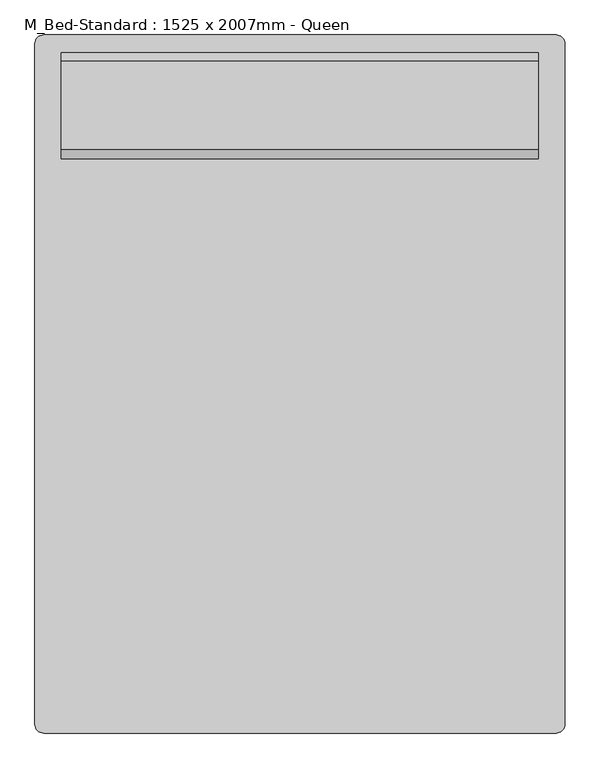
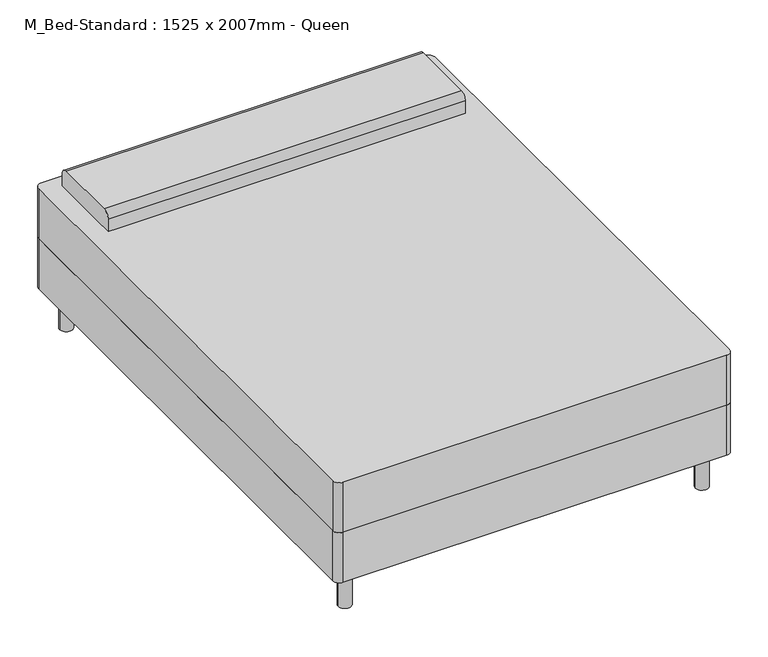
"""IFC4 building model written with IfcOpenShell, lengths in millimetres: furniture geometry, M_Bed-Standard : 1525 x 2007mm - Queen."""

import ifcopenshell
import ifcopenshell.guid

model = None  # the IFC model being written
_history = None  # IfcOwnerHistory: only IFC2X3 demands one
_inside = {}  # id of a spatial element -> (the spatial element, [elements in it])
_under = {}  # id of a project, library or spatial element -> (it, [spatial elements below it])
_declared = {}  # id of a project -> (the project, [libraries it declares])
_typed = {}  # id of a type object -> (the type object, [elements of that type])
_made_of = {}  # id of a material, layer set ... -> (it, [elements and type objects made of it])


def new_model(schema):
    """Start an empty IFC model of exactly this schema.

    Asked for "IFC4X3", IfcOpenShell would pick the latest addendum, in which some entities
    have other attributes; the version numbers below select the first issue.
    IFC2X3 requires an IfcOwnerHistory on every rooted entity: one is made here for all.
    """
    global model, _history
    if schema == "IFC4X3":
        model = ifcopenshell.file(schema_version=(4, 3, 0, 0))
    else:
        model = ifcopenshell.file(schema=schema)
    _inside.clear()
    _under.clear()
    _declared.clear()
    _typed.clear()
    _made_of.clear()
    _history = None
    if model.schema == "IFC2X3":
        org = make("IfcOrganization", Name="unknown")
        user = make(
            "IfcPersonAndOrganization",
            ThePerson=make("IfcPerson", FamilyName="unknown"),
            TheOrganization=org,
        )
        app = make(
            "IfcApplication",
            ApplicationDeveloper=org,
            Version="unknown",
            ApplicationFullName="unknown",
            ApplicationIdentifier="unknown",
        )
        _history = make(
            "IfcOwnerHistory",
            OwningUser=user,
            OwningApplication=app,
            ChangeAction="ADDED",
            CreationDate=0,
        )
    return model


def make(cls, **values):
    """One entity of the class cls with the attributes given. An attribute that is None is left unset."""
    return model.create_entity(
        cls, **{name: value for name, value in values.items() if value is not None}
    )


def rooted(cls, **values):
    """An entity with a GlobalId (a new one), such as an element, a storey or a relation."""
    return make(cls, GlobalId=ifcopenshell.guid.new(), OwnerHistory=_history, **values)


def si_unit(unit_type, name, prefix=None):
    """IfcSIUnit, for example si_unit("LENGTHUNIT", "METRE", prefix="MILLI")."""
    return make("IfcSIUnit", UnitType=unit_type, Prefix=prefix, Name=name)


def assignment(units):
    """IfcUnitAssignment: the units of a project."""
    return None if units is None else make("IfcUnitAssignment", Units=units)


def point(xyz):
    """IfcCartesianPoint."""
    return None if xyz is None else make("IfcCartesianPoint", Coordinates=xyz)


def direction(xyz):
    """IfcDirection."""
    return None if xyz is None else make("IfcDirection", DirectionRatios=xyz)


def frame(location, z_axis=None, x_axis=None):
    """IfcAxis2Placement3D, a coordinate frame: its origin and axes. An axis left out is left unset."""
    return make(
        "IfcAxis2Placement3D",
        Location=point(location),
        Axis=direction(z_axis),
        RefDirection=direction(x_axis),
    )


def frame_2d(location, x_axis=None):
    """IfcAxis2Placement2D, a coordinate frame in the plane: its origin and x axis."""
    return make(
        "IfcAxis2Placement2D", Location=point(location), RefDirection=direction(x_axis)
    )


def origin():
    """The frame at (0, 0, 0) with its axes left unset."""
    return frame((0.0, 0.0, 0.0))


def origin_with_axes():
    """The frame at (0, 0, 0) with the z axis (0, 0, 1) and the x axis (1, 0, 0) written out."""
    return frame((0.0, 0.0, 0.0), z_axis=(0.0, 0.0, 1.0), x_axis=(1.0, 0.0, 0.0))


def place(relative_to, where):
    """IfcLocalPlacement: puts the frame where relative to a parent placement (None: the world)."""
    return make(
        "IfcLocalPlacement", PlacementRelTo=relative_to, RelativePlacement=where
    )


def context(
    kind, dimensions, precision=None, world=None, true_north=None, identifier=None
):
    """IfcGeometricRepresentationContext, for example the 3D "Model" context."""
    return make(
        "IfcGeometricRepresentationContext",
        ContextIdentifier=identifier,
        ContextType=kind,
        CoordinateSpaceDimension=dimensions,
        Precision=precision,
        WorldCoordinateSystem=world,
        TrueNorth=true_north,
    )


def project(units=None, contexts=None):
    """IfcProject with its units and contexts."""
    return rooted(
        "IfcProject",
        Name="project",
        RepresentationContexts=contexts,
        UnitsInContext=assignment(units),
    )


def spatial(cls, under=None, at=None, **own):
    """A site, building, storey or space (cls), placed at a placement, below another one or the project."""
    s = rooted(cls, ObjectPlacement=at, **own)
    if under is not None:
        _under.setdefault(under.id(), (under, []))[1].append(s)
    return s


def polyline(points):
    """IfcPolyline through the points."""
    return make("IfcPolyline", Points=[point(p) for p in points])


def circle_curve(where, radius):
    """IfcCircle in the frame where."""
    return make("IfcCircle", Position=where, Radius=radius)


def trimmed(basis, trim1, trim2, sense, master):
    """IfcTrimmedCurve: the piece of a basis curve between two trims."""
    return make(
        "IfcTrimmedCurve",
        BasisCurve=basis,
        Trim1=trim1,
        Trim2=trim2,
        SenseAgreement=sense,
        MasterRepresentation=master,
    )


def segment(curve, same_sense, transition):
    """IfcCompositeCurveSegment."""
    return make(
        "IfcCompositeCurveSegment",
        Transition=transition,
        SameSense=same_sense,
        ParentCurve=curve,
    )


def composite_curve(segments, self_intersect=None):
    """IfcCompositeCurve: segments joined end to end."""
    return make("IfcCompositeCurve", Segments=segments, SelfIntersect=self_intersect)


def outline(outer, holes=None, kind="AREA"):
    """IfcArbitraryClosedProfileDef: a profile drawn as a closed curve; with holes, ...WithVoids."""
    if holes is None:
        return make("IfcArbitraryClosedProfileDef", ProfileType=kind, OuterCurve=outer)
    return make(
        "IfcArbitraryProfileDefWithVoids",
        ProfileType=kind,
        OuterCurve=outer,
        InnerCurves=holes,
    )


def extrude(swept, where, along, depth):
    """IfcExtrudedAreaSolid: the profile swept, set in the frame where, extruded along a direction by depth."""
    return make(
        "IfcExtrudedAreaSolid",
        SweptArea=swept,
        Position=where,
        ExtrudedDirection=direction(along),
        Depth=depth,
    )


def shape(context_of_items, identifier, shape_type, items):
    """IfcShapeRepresentation: the items that make up one representation, for example the "Body"."""
    return make(
        "IfcShapeRepresentation",
        ContextOfItems=context_of_items,
        RepresentationIdentifier=identifier,
        RepresentationType=shape_type,
        Items=items,
    )


def source(mapping_origin, context_of_items, identifier, shape_type, items):
    """IfcRepresentationMap: a shape defined once, which mapped items show again and again."""
    return make(
        "IfcRepresentationMap",
        MappingOrigin=mapping_origin,
        MappedRepresentation=shape(context_of_items, identifier, shape_type, items),
    )


def transform(
    local_origin,
    x_axis=None,
    y_axis=None,
    z_axis=None,
    scale=None,
    scale2=None,
    scale3=None,
    uniform=True,
):
    """IfcCartesianTransformationOperator3D, or its non-uniform kind. x_axis, y_axis, z_axis: its Axis1, 2, 3."""
    if uniform:
        return make(
            "IfcCartesianTransformationOperator3D",
            Axis1=direction(x_axis),
            Axis2=direction(y_axis),
            LocalOrigin=point(local_origin),
            Scale=scale,
            Axis3=direction(z_axis),
        )
    return make(
        "IfcCartesianTransformationOperator3DnonUniform",
        Axis1=direction(x_axis),
        Axis2=direction(y_axis),
        LocalOrigin=point(local_origin),
        Scale=scale,
        Axis3=direction(z_axis),
        Scale2=scale2,
        Scale3=scale3,
    )


def mapped(mapping_source, mapping_target):
    """IfcMappedItem: shows the shape of a source again, moved by a transform."""
    return make(
        "IfcMappedItem", MappingSource=mapping_source, MappingTarget=mapping_target
    )


def made_of(thing, what):
    """Note that an element or type object is made of a material, layer set ...; save() writes the relation."""
    if what is not None:
        _made_of.setdefault(what.id(), (what, []))[1].append(thing)
    return thing


def element(
    cls,
    number,
    at=None,
    inside=None,
    cuts=None,
    type_object=None,
    material=None,
    context=None,
    identifier="Body",
    shape_type=None,
    held_by="IfcProductDefinitionShape",
    body=None,
    shapes=None,
    **own,
):
    """One element of the class cls, such as IfcWall. Its Tag is "e" and its number.

    at: its placement. inside: the storey or other place that contains it. cuts: it is an
    opening in that element (IfcRelVoidsElement). A single representation is given by context,
    identifier, shape_type and body (its items); several are given by shapes. held_by: the class
    of the entity that holds the representations. save() writes the other relations.
    """
    e = rooted(cls, Tag="e%d" % number, ObjectPlacement=at, **own)
    if body is not None:
        shapes = [shape(context, identifier, shape_type, body)]
    if shapes is not None:
        e.Representation = make(held_by, Representations=shapes)
    if inside is not None:
        _inside.setdefault(inside.id(), (inside, []))[1].append(e)
    if cuts is not None:
        rooted(
            "IfcRelVoidsElement", RelatingBuildingElement=cuts, RelatedOpeningElement=e
        )
    if type_object is not None:
        _typed.setdefault(type_object.id(), (type_object, []))[1].append(e)
    return made_of(e, material)


def aggregate(whole, parts):
    """IfcRelAggregates: a whole, such as a stair, and the parts it consists of."""
    return rooted("IfcRelAggregates", RelatingObject=whole, RelatedObjects=parts)


def save(model, path):
    """Write the relations noted so far, then the file.

    IfcRelAggregates (storeys below a building ...), IfcRelContainedInSpatialStructure (elements
    in a storey), IfcRelDefinesByType, IfcRelAssociatesMaterial and IfcRelDeclares: one each for
    every whole, place, type object, material and project.
    """
    for whole, parts in _under.values():
        aggregate(whole, parts)
    for where, things in _inside.values():
        rooted(
            "IfcRelContainedInSpatialStructure",
            RelatedElements=things,
            RelatingStructure=where,
        )
    for kind, things in _typed.values():
        rooted("IfcRelDefinesByType", RelatedObjects=things, RelatingType=kind)
    for what, things in _made_of.values():
        rooted("IfcRelAssociatesMaterial", RelatedObjects=things, RelatingMaterial=what)
    for by, libraries in _declared.values():
        rooted("IfcRelDeclares", RelatingContext=by, RelatedDefinitions=libraries)
    model.write(path)


def m_bed_standard_1525_x_2007mm_queen_67038778(model_context):
    return source(origin(), model_context, "Body", "SweptSolid", [
        extrude(outline(composite_curve([segment(polyline([(-491.0114754, -1023.695082), (-491.0114754, 932.504918)]), True, "CONTINUOUS"), segment(trimmed(circle_curve(frame_2d((-465.6114754, 932.504918)), 25.4), [point((-491.0114754, 932.504918))], [point((-465.6114754, 957.904918))], False, "CARTESIAN"), True, "CONTINUOUS"), segment(polyline([(-465.6114754, 957.904918), (1008.5885246, 957.904918)]), True, "CONTINUOUS"), segment(trimmed(circle_curve(frame_2d((1008.5885246, 932.504918)), 25.4), [point((1008.5885246, 957.904918))], [point((1033.9885246, 932.504918))], False, "CARTESIAN"), True, "CONTINUOUS"), segment(polyline([(1033.9885246, 932.504918), (1033.9885246, -1023.695082)]), True, "CONTINUOUS"), segment(trimmed(circle_curve(frame_2d((1008.5885246, -1023.695082)), 25.4), [point((1033.9885246, -1023.695082))], [point((1008.5885246, -1049.095082))], False, "CARTESIAN"), True, "CONTINUOUS"), segment(polyline([(1008.5885246, -1049.095082), (-465.6114754, -1049.095082)]), True, "CONTINUOUS"), segment(trimmed(circle_curve(frame_2d((-465.6114754, -1023.695082)), 25.4), [point((-465.6114754, -1049.095082))], [point((-491.0114754, -1023.695082))], False, "CARTESIAN"), True, "CONTINUOUS")], self_intersect=False)), frame((0.0, 0.0, 152.4), z_axis=(0.0, 0.0, 1.0), x_axis=(1.0, 0.0, 0.0)), (0.0, 0.0, 1.0), 203.2),
        extrude(outline(composite_curve([segment(polyline([(602.304918, 558.8), (602.304918, 609.6)]), True, "CONTINUOUS"), segment(trimmed(circle_curve(frame_2d((627.704918, 609.6)), 25.4), [point((602.304918, 609.6))], [point((627.704918, 635.0))], False, "CARTESIAN"), True, "CONTINUOUS"), segment(polyline([(627.704918, 635.0), (881.704918, 635.0)]), True, "CONTINUOUS"), segment(trimmed(circle_curve(frame_2d((881.704918, 609.6)), 25.4), [point((881.704918, 635.0))], [point((907.104918, 609.6))], False, "CARTESIAN"), True, "CONTINUOUS"), segment(polyline([(907.104918, 609.6), (907.104918, 558.8), (602.304918, 558.8)]), True, "CONTINUOUS")], self_intersect=False)), frame((-414.8114754, 0.0, 0.0), z_axis=(1.0, 0.0, 0.0), x_axis=(0.0, 1.0, 0.0)), (0.0, 0.0, 1.0), 1372.6),
        extrude(outline(composite_curve([segment(trimmed(circle_curve(frame_2d((-414.8114754, 881.704918)), 25.4), [point((-440.2114754, 881.704918))], [point((-389.4114754, 881.704918))], False, "CARTESIAN"), True, "CONTINUOUS"), segment(trimmed(circle_curve(frame_2d((-414.8114754, 881.704918)), 25.4), [point((-389.4114754, 881.704918))], [point((-440.2114754, 881.704918))], False, "CARTESIAN"), True, "CONTINUOUS")], self_intersect=False)), origin_with_axes(), (0.0, 0.0, 1.0), 152.4),
        extrude(outline(composite_curve([segment(trimmed(circle_curve(frame_2d((957.7885246, 881.704918)), 25.4), [point((932.3885246, 881.704918))], [point((983.1885246, 881.704918))], False, "CARTESIAN"), True, "CONTINUOUS"), segment(trimmed(circle_curve(frame_2d((957.7885246, 881.704918)), 25.4), [point((983.1885246, 881.704918))], [point((932.3885246, 881.704918))], False, "CARTESIAN"), True, "CONTINUOUS")], self_intersect=False)), origin_with_axes(), (0.0, 0.0, 1.0), 152.4),
        extrude(outline(composite_curve([segment(trimmed(circle_curve(frame_2d((957.7885246, -972.895082)), 25.4), [point((932.3885246, -972.895082))], [point((983.1885246, -972.895082))], False, "CARTESIAN"), True, "CONTINUOUS"), segment(trimmed(circle_curve(frame_2d((957.7885246, -972.895082)), 25.4), [point((983.1885246, -972.895082))], [point((932.3885246, -972.895082))], False, "CARTESIAN"), True, "CONTINUOUS")], self_intersect=False)), origin_with_axes(), (0.0, 0.0, 1.0), 152.4),
        extrude(outline(composite_curve([segment(trimmed(circle_curve(frame_2d((-414.8114754, -972.895082)), 25.4), [point((-440.2114754, -972.895082))], [point((-389.4114754, -972.895082))], False, "CARTESIAN"), True, "CONTINUOUS"), segment(trimmed(circle_curve(frame_2d((-414.8114754, -972.895082)), 25.4), [point((-389.4114754, -972.895082))], [point((-440.2114754, -972.895082))], False, "CARTESIAN"), True, "CONTINUOUS")], self_intersect=False)), origin_with_axes(), (0.0, 0.0, 1.0), 152.4),
        extrude(outline(composite_curve([segment(polyline([(-465.6114754, 957.904918), (1008.5885246, 957.904918)]), True, "CONTINUOUS"), segment(trimmed(circle_curve(frame_2d((1008.5885246, 932.504918)), 25.4), [point((1008.5885246, 957.904918))], [point((1033.9885246, 932.504918))], False, "CARTESIAN"), True, "CONTINUOUS"), segment(polyline([(1033.9885246, 932.504918), (1033.9885246, -1023.695082)]), True, "CONTINUOUS"), segment(trimmed(circle_curve(frame_2d((1008.5885246, -1023.695082)), 25.4), [point((1033.9885246, -1023.695082))], [point((1008.5885246, -1049.095082))], False, "CARTESIAN"), True, "CONTINUOUS"), segment(polyline([(1008.5885246, -1049.095082), (-465.6114754, -1049.095082)]), True, "CONTINUOUS"), segment(trimmed(circle_curve(frame_2d((-465.6114754, -1023.695082)), 25.4), [point((-465.6114754, -1049.095082))], [point((-491.0114754, -1023.695082))], False, "CARTESIAN"), True, "CONTINUOUS"), segment(polyline([(-491.0114754, -1023.695082), (-491.0114754, 932.504918)]), True, "CONTINUOUS"), segment(trimmed(circle_curve(frame_2d((-465.6114754, 932.504918)), 25.4), [point((-491.0114754, 932.504918))], [point((-465.6114754, 957.904918))], False, "CARTESIAN"), True, "CONTINUOUS")], self_intersect=False)), frame((0.0, 0.0, 355.6), z_axis=(0.0, 0.0, 1.0), x_axis=(1.0, 0.0, 0.0)), (0.0, 0.0, 1.0), 203.2),
    ])


if __name__ == "__main__":
    model = new_model("IFC4")
    model_context = context("Model", 3, world=origin())
    ifc_project = project(units=[si_unit("LENGTHUNIT", "METRE", prefix="MILLI")], contexts=[model_context])
    site = spatial("IfcSite", under=ifc_project)
    building = spatial("IfcBuilding", under=site)
    placement = place(None, origin())
    m_bed_standard_1525_x_2007mm_queen_shape = m_bed_standard_1525_x_2007mm_queen_67038778(model_context)
    element("IfcFurniture", 1, ObjectType="M_Bed-Standard : 1525 x 2007mm - Queen", at=placement, inside=building, context=model_context, shape_type="MappedRepresentation", body=[
        mapped(m_bed_standard_1525_x_2007mm_queen_shape, transform((0.0, 0.0, 0.0), x_axis=(1.0, 0.0, 0.0), y_axis=(0.0, 1.0, 0.0), z_axis=(0.0, 0.0, 1.0))),
    ])
    save(model, "model.ifc")

# Revit data of these elements
# Type "M_Bed-Standard : 1525 x 2007mm - Queen"
#   Manufacturer = "Manufacturer"
#   AccessibilityPerformance = "AccessibilityPerformance"
#   CodePerformance = "CodePerformance"
#   Area = "Area"
#   Color = "Color"
#   Constituents = "Constituents"
#   Features = "Features"
#   Finish = "Finish"
#   Grade = "Grade"
#   Material = "Material"
#   ModelReference = "ModelReference"
#   NominalHeight = "NominalHeight"
#   NominalLength = "NominalLength"
#   NominalWidth = "NominalWidth"
#   ProductionYear = "ProductionYear"
#   Reference = "Reference"
#   Shape = "Shape"
#   Size = "Size"
#   SustainabilityPerformance = "SustainabilityPerformance"
#   WarrantyDescription = "WarrantyDescription"
#   WarrantyDurationLabor = "WarrantyDurationLabor"
#   WarrantyDurationParts = "WarrantyDurationParts"
#   WarrantyGuarantorLabor = "WarrantyGuarantorLabor"
#   WarrantyGuarantorParts = "WarrantyGuarantorParts"
#   ExpectedLife = "ExpectedLife"
#   ReplacementCost = "ReplacementCost"
#   AssetAccountingType = "NONFIXED"
#   ModelLabel = "ModelLabel"
#   Length = 2.007 m
#   Width = 1.525 m
#   Leg Material = Metal - Chrome
#   Mattress Material = Textile - White
# Element 1 (IfcFurniture, "M_Bed-Standard : 1525 x 2007mm - Queen")
#   Materials on its faces: "Textile - White", "Metal - Chrome"
# Materials
#   "Metal - Chrome": class "Metal", colour RGB 17 17 17, transparency 0
#   "Textile - White": class "Fabric", colour RGB 247 247 239, transparency 0
